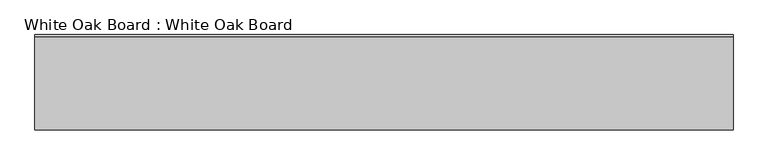
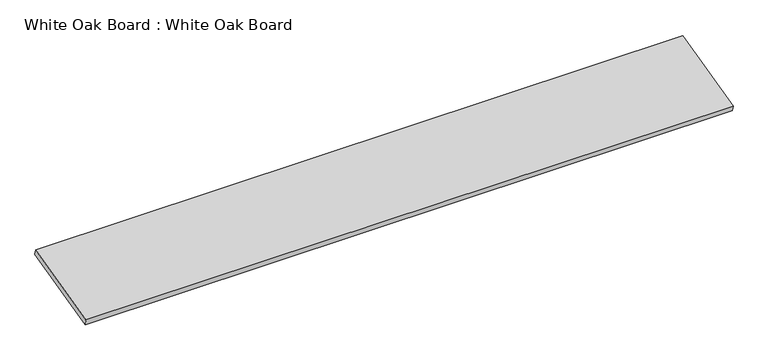
"""IFC4 building model written with IfcOpenShell, lengths in millimetres: proxy geometry, White Oak Board : White Oak Board."""

from ifc_helpers import new_model, si_unit, frame, origin, place, context, project, spatial, polyline, outline, extrude, source, transform, mapped, element, save


def white_oak_board_white_oak_board_d3a0b81f(model_context):
    return source(origin(), model_context, "Body", "SweptSolid", [
        extrude(outline(polyline([(0.0, -276.86), (0.0, 0.0), (2000.25, 0.0), (2000.25, -276.86), (0.0, -276.86)])), frame((12382.7678845, -5313.3122874, 42390.9228742), z_axis=(0.0, -0.24292009113324656, 0.9700463026700402), x_axis=(1.0, 0.0, 0.0)), (0.0, 0.0, 1.0), 19.05),
    ])


if __name__ == "__main__":
    model = new_model("IFC4")
    model_context = context("Model", 3, world=origin())
    ifc_project = project(units=[si_unit("LENGTHUNIT", "METRE", prefix="MILLI")], contexts=[model_context])
    site = spatial("IfcSite", under=ifc_project)
    building = spatial("IfcBuilding", under=site)
    placement = place(None, origin())
    white_oak_board_white_oak_board_shape = white_oak_board_white_oak_board_d3a0b81f(model_context)
    element("IfcBuildingElementProxy", 1, Name="White Oak Board : White Oak Board", ObjectType="White Oak Board : White Oak Board", at=placement, inside=building, context=model_context, shape_type="MappedRepresentation", body=[
        mapped(white_oak_board_white_oak_board_shape, transform((0.0, 0.0, 0.0), x_axis=(1.0, 0.0, 0.0), y_axis=(0.0, 1.0, 0.0), z_axis=(0.0, 0.0, 1.0))),
    ])
    save(model, "model.ifc")

# Revit data of these elements
# Type "White Oak Board : White Oak Board"
#   NameOverride = "White Oak Board"
# Element 1 (IfcBuildingElementProxy, "White Oak Board : White Oak Board")
#   Materials on its faces: "WHITE OAK (SPEC T.B.D.) OVER BUILDING WRAP"
# Materials
#   "WHITE OAK (SPEC T.B.D.) OVER BUILDING WRAP": class "Unassigned", colour RGB 227 188 136, transparency 0, Cost = 0
